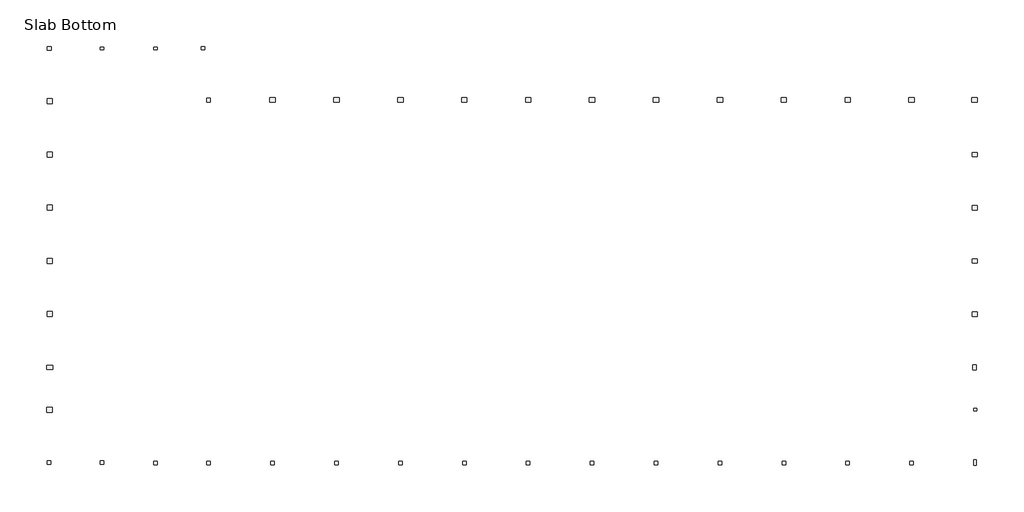
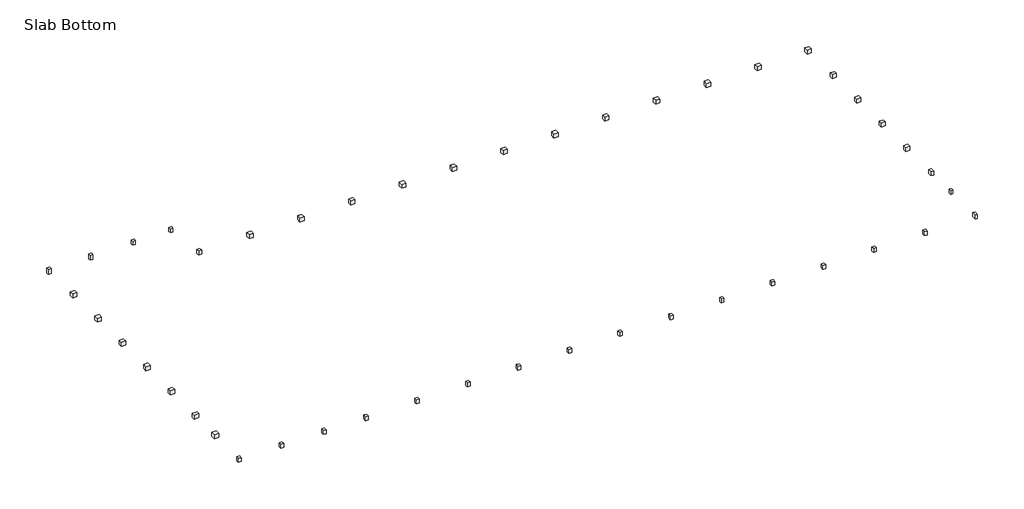
# One storey: 46 slabs.
"""IFC4 building model written with IfcOpenShell, lengths in millimetres."""

from ifc_helpers import new_model, si_unit, frame, origin, place, context, project, spatial, polyline, outline, extrude, faceted_brep, element, save

model = new_model("IFC4")

# Units and contexts
model_context = context("Model", 3, world=origin())
ifc_project = project(units=[si_unit("LENGTHUNIT", "METRE", prefix="MILLI")], contexts=[model_context])

# Site, building, storey
site = spatial("IfcSite", under=ifc_project)
building = spatial("IfcBuilding", under=site)
storey = spatial("IfcBuildingStorey", under=building, Name="Slab Bottom", Elevation=-152.4)

# Slabs
placement = place(None, origin())
element("IfcSlab", 1, ObjectType="Footing-Rectangular : P1", at=placement, inside=storey, context=model_context, shape_type="SweptSolid", body=[
    extrude(outline(polyline([(411310.2398264, -572441.1413841), (411615.0398264, -572441.1413841), (411615.0398264, -572745.9413841), (411310.2398264, -572745.9413841), (411310.2398264, -572441.1413841)])), frame((0.0, 0.0, -914.4), z_axis=(0.0, 0.0, 1.0), x_axis=(1.0, 0.0, 0.0)), (0.0, 0.0, 1.0), 609.6),
])
element("IfcSlab", 2, ObjectType="Footing-Rectangular : P10", at=placement, inside=storey, context=model_context, shape_type="SweptSolid", body=[
    extrude(outline(polyline([(304585.7898264, -567919.9413841), (304585.7898264, -567462.7413841), (305271.5898264, -567462.7413841), (305271.5898264, -567919.9413841), (304585.7898264, -567919.9413841)])), frame((0.0, 0.0, -914.4), z_axis=(0.0, 0.0, 1.0), x_axis=(1.0, 0.0, 0.0)), (0.0, 0.0, 1.0), 609.6),
])
element("IfcSlab", 3, ObjectType="Footing-Rectangular : P11", at=placement, inside=storey, context=model_context, shape_type="SweptSolid", body=[
    extrude(outline(polyline([(411138.7898264, -549562.0913841), (411138.7898264, -549054.0913841), (411697.5898264, -549054.0913841), (411697.5898264, -549562.0913841), (411138.7898264, -549562.0913841)])), frame((0.0, 0.0, -914.4), z_axis=(0.0, 0.0, 1.0), x_axis=(1.0, 0.0, 0.0)), (0.0, 0.0, 1.0), 609.6),
])
element("IfcSlab", 4, ObjectType="Footing-Rectangular : P11A", at=placement, inside=storey, context=model_context, shape_type="SweptSolid", body=[
    extrude(outline(polyline([(411138.7898264, -561817.5913841), (411138.7898264, -561309.5913841), (411697.5898264, -561309.5913841), (411697.5898264, -561817.5913841), (411138.7898264, -561817.5913841)])), frame((0.0, 0.0, -914.4), z_axis=(0.0, 0.0, 1.0), x_axis=(1.0, 0.0, 0.0)), (0.0, 0.0, 1.0), 609.6),
])
element("IfcSlab", 5, ObjectType="Footing-Rectangular : P12", at=placement, inside=storey, context=model_context, shape_type="SweptSolid", body=[
    extrude(outline(polyline([(304649.2898264, -537331.9913841), (304649.2898264, -536773.1913841), (305258.8898264, -536773.1913841), (305258.8898264, -537331.9913841), (304649.2898264, -537331.9913841)])), frame((0.0, 0.0, -914.4), z_axis=(0.0, 0.0, 1.0), x_axis=(1.0, 0.0, 0.0)), (0.0, 0.0, 1.0), 609.6),
])
element("IfcSlab", 6, ObjectType="Footing-Rectangular : P12", at=placement, inside=storey, context=model_context, shape_type="SweptSolid", body=[
    extrude(outline(polyline([(304649.2898264, -543459.7413841), (304649.2898264, -542900.9413841), (305258.8898264, -542900.9413841), (305258.8898264, -543459.7413841), (304649.2898264, -543459.7413841)])), frame((0.0, 0.0, -914.4), z_axis=(0.0, 0.0, 1.0), x_axis=(1.0, 0.0, 0.0)), (0.0, 0.0, 1.0), 609.6),
])
element("IfcSlab", 7, ObjectType="Footing-Rectangular : P12", at=placement, inside=storey, context=model_context, shape_type="SweptSolid", body=[
    extrude(outline(polyline([(304649.2898264, -549587.4913841), (304649.2898264, -549028.6913841), (305258.8898264, -549028.6913841), (305258.8898264, -549587.4913841), (304649.2898264, -549587.4913841)])), frame((0.0, 0.0, -914.4), z_axis=(0.0, 0.0, 1.0), x_axis=(1.0, 0.0, 0.0)), (0.0, 0.0, 1.0), 609.6),
])
element("IfcSlab", 8, ObjectType="Footing-Rectangular : P12", at=placement, inside=storey, context=model_context, shape_type="SweptSolid", body=[
    extrude(outline(polyline([(304649.2898264, -555715.2413841), (304649.2898264, -555156.4413841), (305258.8898264, -555156.4413841), (305258.8898264, -555715.2413841), (304649.2898264, -555715.2413841)])), frame((0.0, 0.0, -914.4), z_axis=(0.0, 0.0, 1.0), x_axis=(1.0, 0.0, 0.0)), (0.0, 0.0, 1.0), 609.6),
])
element("IfcSlab", 9, ObjectType="Footing-Rectangular : P12", at=placement, inside=storey, context=model_context, shape_type="SweptSolid", body=[
    extrude(outline(polyline([(304649.2898264, -561842.9913841), (304649.2898264, -561284.1913841), (305258.8898264, -561284.1913841), (305258.8898264, -561842.9913841), (304649.2898264, -561842.9913841)])), frame((0.0, 0.0, -914.4), z_axis=(0.0, 0.0, 1.0), x_axis=(1.0, 0.0, 0.0)), (0.0, 0.0, 1.0), 609.6),
])
element("IfcSlab", 10, ObjectType="Footing-Rectangular : P13", at=placement, inside=storey, context=model_context, shape_type="SweptSolid", body=[
    extrude(outline(polyline([(396476.6398264, -536627.1413358), (397086.2398264, -536627.1413358), (397086.2398264, -537185.9413358), (396476.6398264, -537185.9413358), (396476.6398264, -536627.1413358)])), frame((0.0, 0.0, -914.4), z_axis=(0.0, 0.0, 1.0), x_axis=(1.0, 0.0, 0.0)), (0.0, 0.0, 1.0), 609.6),
])
element("IfcSlab", 11, ObjectType="Footing-Rectangular : P13", at=placement, inside=storey, context=model_context, shape_type="SweptSolid", body=[
    extrude(outline(polyline([(389123.3398264, -536627.1413358), (389732.9398264, -536627.1413358), (389732.9398264, -537185.9413358), (389123.3398264, -537185.9413358), (389123.3398264, -536627.1413358)])), frame((0.0, 0.0, -914.4), z_axis=(0.0, 0.0, 1.0), x_axis=(1.0, 0.0, 0.0)), (0.0, 0.0, 1.0), 609.6),
])
element("IfcSlab", 12, ObjectType="Footing-Rectangular : P13", at=placement, inside=storey, context=model_context, shape_type="SweptSolid", body=[
    extrude(outline(polyline([(381770.0398264, -536627.1413358), (382379.6398264, -536627.1413358), (382379.6398264, -537185.9413358), (381770.0398264, -537185.9413358), (381770.0398264, -536627.1413358)])), frame((0.0, 0.0, -914.4), z_axis=(0.0, 0.0, 1.0), x_axis=(1.0, 0.0, 0.0)), (0.0, 0.0, 1.0), 609.6),
])
element("IfcSlab", 13, ObjectType="Footing-Rectangular : P13", at=placement, inside=storey, context=model_context, shape_type="SweptSolid", body=[
    extrude(outline(polyline([(374416.7398264, -536627.1413358), (375026.3398264, -536627.1413358), (375026.3398264, -537185.9413358), (374416.7398264, -537185.9413358), (374416.7398264, -536627.1413358)])), frame((0.0, 0.0, -914.4), z_axis=(0.0, 0.0, 1.0), x_axis=(1.0, 0.0, 0.0)), (0.0, 0.0, 1.0), 609.6),
])
element("IfcSlab", 14, ObjectType="Footing-Rectangular : P13", at=placement, inside=storey, context=model_context, shape_type="SweptSolid", body=[
    extrude(outline(polyline([(367063.4398264, -536627.1413358), (367673.0398264, -536627.1413358), (367673.0398264, -537185.9413358), (367063.4398264, -537185.9413358), (367063.4398264, -536627.1413358)])), frame((0.0, 0.0, -914.4), z_axis=(0.0, 0.0, 1.0), x_axis=(1.0, 0.0, 0.0)), (0.0, 0.0, 1.0), 609.6),
])
element("IfcSlab", 15, ObjectType="Footing-Rectangular : P13", at=placement, inside=storey, context=model_context, shape_type="SweptSolid", body=[
    extrude(outline(polyline([(359710.1398264, -536627.1413358), (360319.7398264, -536627.1413358), (360319.7398264, -537185.9413358), (359710.1398264, -537185.9413358), (359710.1398264, -536627.1413358)])), frame((0.0, 0.0, -914.4), z_axis=(0.0, 0.0, 1.0), x_axis=(1.0, 0.0, 0.0)), (0.0, 0.0, 1.0), 609.6),
])
element("IfcSlab", 16, ObjectType="Footing-Rectangular : P13", at=placement, inside=storey, context=model_context, shape_type="SweptSolid", body=[
    extrude(outline(polyline([(352356.8398264, -536627.1413358), (352966.4398264, -536627.1413358), (352966.4398264, -537185.9413358), (352356.8398264, -537185.9413358), (352356.8398264, -536627.1413358)])), frame((0.0, 0.0, -914.4), z_axis=(0.0, 0.0, 1.0), x_axis=(1.0, 0.0, 0.0)), (0.0, 0.0, 1.0), 609.6),
])
element("IfcSlab", 17, ObjectType="Footing-Rectangular : P13", at=placement, inside=storey, context=model_context, shape_type="SweptSolid", body=[
    extrude(outline(polyline([(345003.5398264, -536627.1413358), (345613.1398264, -536627.1413358), (345613.1398264, -537185.9413358), (345003.5398264, -537185.9413358), (345003.5398264, -536627.1413358)])), frame((0.0, 0.0, -914.4), z_axis=(0.0, 0.0, 1.0), x_axis=(1.0, 0.0, 0.0)), (0.0, 0.0, 1.0), 609.6),
])
element("IfcSlab", 18, ObjectType="Footing-Rectangular : P13", at=placement, inside=storey, context=model_context, shape_type="SweptSolid", body=[
    extrude(outline(polyline([(337650.2398264, -536627.1413358), (338259.8398264, -536627.1413358), (338259.8398264, -537185.9413358), (337650.2398264, -537185.9413358), (337650.2398264, -536627.1413358)])), frame((0.0, 0.0, -914.4), z_axis=(0.0, 0.0, 1.0), x_axis=(1.0, 0.0, 0.0)), (0.0, 0.0, 1.0), 609.6),
])
element("IfcSlab", 19, ObjectType="Footing-Rectangular : P13", at=placement, inside=storey, context=model_context, shape_type="SweptSolid", body=[
    extrude(outline(polyline([(330296.9398264, -536627.1413358), (330906.5398264, -536627.1413358), (330906.5398264, -537185.9413358), (330296.9398264, -537185.9413358), (330296.9398264, -536627.1413358)])), frame((0.0, 0.0, -914.4), z_axis=(0.0, 0.0, 1.0), x_axis=(1.0, 0.0, 0.0)), (0.0, 0.0, 1.0), 609.6),
])
element("IfcSlab", 20, ObjectType="Footing-Rectangular : P13A", at=placement, inside=storey, context=model_context, shape_type="SweptSolid", body=[
    extrude(outline(polyline([(411081.6397781, -536620.7913358), (411691.2397781, -536620.7913358), (411691.2397781, -537179.5913358), (411081.6397781, -537179.5913358), (411081.6397781, -536620.7913358)])), frame((0.0, 0.0, -914.4), z_axis=(0.0, 0.0, 1.0), x_axis=(1.0, 0.0, 0.0)), (0.0, 0.0, 1.0), 609.6),
])
element("IfcSlab", 21, ObjectType="Footing-Rectangular : P13B", at=placement, inside=storey, context=model_context, shape_type="SweptSolid", body=[
    extrude(outline(polyline([(403829.9398264, -536627.1413358), (404439.5398264, -536627.1413358), (404439.5398264, -537185.9413358), (403829.9398264, -537185.9413358), (403829.9398264, -536627.1413358)])), frame((0.0, 0.0, -914.4), z_axis=(0.0, 0.0, 1.0), x_axis=(1.0, 0.0, 0.0)), (0.0, 0.0, 1.0), 609.6),
])
element("IfcSlab", 22, ObjectType="Footing-Rectangular : P14", at=placement, inside=storey, context=model_context, shape_type="Brep", body=[
    faceted_brep([(304598.4898264, -572288.7413841, -304.8), (304598.4898264, -572898.3413841, -304.8), (305258.8898264, -572898.3413841, -304.8), (305258.8898264, -572810.8391729, -304.8), (305258.8898264, -572404.4391729, -304.8), (305258.8898264, -572288.7413841, -304.8), (304598.4898264, -572288.7413841, -914.4), (304598.4898264, -572898.3413841, -914.4), (305258.8898264, -572898.3413841, -914.4), (305258.8898264, -572288.7413841, -914.4)], [[[0, 1, 2, 3, 4, 5]], [[1, 0, 6, 7]], [[2, 1, 7, 8]], [[5, 4, 3, 2, 8, 9]], [[0, 5, 9, 6]], [[7, 6, 9, 8]]]),
])
element("IfcSlab", 23, ObjectType="Footing-Rectangular : P2", at=placement, inside=storey, context=model_context, shape_type="SweptSolid", body=[
    extrude(outline(polyline([(322772.1898264, -530797.8413841), (322772.1898264, -531102.6413841), (322365.7898264, -531102.6413841), (322365.7898264, -530797.8413841), (322772.1898264, -530797.8413841)])), frame((0.0, 0.0, -914.4), z_axis=(0.0, 0.0, 1.0), x_axis=(1.0, 0.0, 0.0)), (0.0, 0.0, 1.0), 609.6),
])
element("IfcSlab", 24, ObjectType="Footing-Rectangular : P3", at=placement, inside=storey, context=model_context, shape_type="SweptSolid", body=[
    extrude(outline(polyline([(411284.8398264, -578384.7413841), (411589.6398264, -578384.7413841), (411589.6398264, -578994.3413841), (411284.8398264, -578994.3413841), (411284.8398264, -578384.7413841)])), frame((0.0, 0.0, -914.4), z_axis=(0.0, 0.0, 1.0), x_axis=(1.0, 0.0, 0.0)), (0.0, 0.0, 1.0), 609.6),
])
element("IfcSlab", 25, ObjectType="Footing-Rectangular : P4", at=placement, inside=storey, context=model_context, shape_type="SweptSolid", body=[
    extrude(outline(polyline([(310789.7398264, -531108.9913841), (310789.7398264, -530804.1913841), (311196.1398264, -530804.1913841), (311196.1398264, -531108.9913841), (310789.7398264, -531108.9913841)])), frame((0.0, 0.0, -1066.8), z_axis=(0.0, 0.0, 1.0), x_axis=(1.0, 0.0, 0.0)), (0.0, 0.0, 1.0), 762.0),
])
element("IfcSlab", 26, ObjectType="Footing-Rectangular : P4", at=placement, inside=storey, context=model_context, shape_type="SweptSolid", body=[
    extrude(outline(polyline([(317323.8898264, -531108.9913841), (316917.4898264, -531108.9913841), (316917.4898264, -530804.1913841), (317323.8898264, -530804.1913841), (317323.8898264, -531108.9913841)])), frame((0.0, 0.0, -914.4), z_axis=(0.0, 0.0, 1.0), x_axis=(1.0, 0.0, 0.0)), (0.0, 0.0, 1.0), 609.6),
])
element("IfcSlab", 27, ObjectType="Footing-Rectangular : P5", at=placement, inside=storey, context=model_context, shape_type="SweptSolid", body=[
    extrude(outline(polyline([(330398.5398264, -578537.1413841), (330804.9398264, -578537.1413841), (330804.9398264, -578943.5413841), (330398.5398264, -578943.5413841), (330398.5398264, -578537.1413841)])), frame((0.0, 0.0, -914.4), z_axis=(0.0, 0.0, 1.0), x_axis=(1.0, 0.0, 0.0)), (0.0, 0.0, 1.0), 609.6),
])
element("IfcSlab", 28, ObjectType="Footing-Rectangular : P5", at=placement, inside=storey, context=model_context, shape_type="SweptSolid", body=[
    extrude(outline(polyline([(337751.8398264, -578537.1413841), (338158.2398264, -578537.1413841), (338158.2398264, -578943.5413841), (337751.8398264, -578943.5413841), (337751.8398264, -578537.1413841)])), frame((0.0, 0.0, -914.4), z_axis=(0.0, 0.0, 1.0), x_axis=(1.0, 0.0, 0.0)), (0.0, 0.0, 1.0), 609.6),
])
element("IfcSlab", 29, ObjectType="Footing-Rectangular : P5", at=placement, inside=storey, context=model_context, shape_type="SweptSolid", body=[
    extrude(outline(polyline([(345105.1398264, -578537.1413841), (345511.5398264, -578537.1413841), (345511.5398264, -578943.5413841), (345105.1398264, -578943.5413841), (345105.1398264, -578537.1413841)])), frame((0.0, 0.0, -914.4), z_axis=(0.0, 0.0, 1.0), x_axis=(1.0, 0.0, 0.0)), (0.0, 0.0, 1.0), 609.6),
])
element("IfcSlab", 30, ObjectType="Footing-Rectangular : P5", at=placement, inside=storey, context=model_context, shape_type="SweptSolid", body=[
    extrude(outline(polyline([(352458.4398264, -578537.1413841), (352864.8398264, -578537.1413841), (352864.8398264, -578943.5413841), (352458.4398264, -578943.5413841), (352458.4398264, -578537.1413841)])), frame((0.0, 0.0, -914.4), z_axis=(0.0, 0.0, 1.0), x_axis=(1.0, 0.0, 0.0)), (0.0, 0.0, 1.0), 609.6),
])
element("IfcSlab", 31, ObjectType="Footing-Rectangular : P5", at=placement, inside=storey, context=model_context, shape_type="SweptSolid", body=[
    extrude(outline(polyline([(359811.7398264, -578537.1413841), (360218.1398264, -578537.1413841), (360218.1398264, -578943.5413841), (359811.7398264, -578943.5413841), (359811.7398264, -578537.1413841)])), frame((0.0, 0.0, -914.4), z_axis=(0.0, 0.0, 1.0), x_axis=(1.0, 0.0, 0.0)), (0.0, 0.0, 1.0), 609.6),
])
element("IfcSlab", 32, ObjectType="Footing-Rectangular : P5", at=placement, inside=storey, context=model_context, shape_type="SweptSolid", body=[
    extrude(outline(polyline([(367165.0398264, -578537.1413841), (367571.4398264, -578537.1413841), (367571.4398264, -578943.5413841), (367165.0398264, -578943.5413841), (367165.0398264, -578537.1413841)])), frame((0.0, 0.0, -914.4), z_axis=(0.0, 0.0, 1.0), x_axis=(1.0, 0.0, 0.0)), (0.0, 0.0, 1.0), 609.6),
])
element("IfcSlab", 33, ObjectType="Footing-Rectangular : P5", at=placement, inside=storey, context=model_context, shape_type="SweptSolid", body=[
    extrude(outline(polyline([(374518.3398264, -578537.1413841), (374924.7398264, -578537.1413841), (374924.7398264, -578943.5413841), (374518.3398264, -578943.5413841), (374518.3398264, -578537.1413841)])), frame((0.0, 0.0, -914.4), z_axis=(0.0, 0.0, 1.0), x_axis=(1.0, 0.0, 0.0)), (0.0, 0.0, 1.0), 609.6),
])
element("IfcSlab", 34, ObjectType="Footing-Rectangular : P5", at=placement, inside=storey, context=model_context, shape_type="SweptSolid", body=[
    extrude(outline(polyline([(381871.6398264, -578537.1413841), (382278.0398264, -578537.1413841), (382278.0398264, -578943.5413841), (381871.6398264, -578943.5413841), (381871.6398264, -578537.1413841)])), frame((0.0, 0.0, -914.4), z_axis=(0.0, 0.0, 1.0), x_axis=(1.0, 0.0, 0.0)), (0.0, 0.0, 1.0), 609.6),
])
element("IfcSlab", 35, ObjectType="Footing-Rectangular : P5", at=placement, inside=storey, context=model_context, shape_type="SweptSolid", body=[
    extrude(outline(polyline([(389224.9398264, -578537.1413841), (389631.3398264, -578537.1413841), (389631.3398264, -578943.5413841), (389224.9398264, -578943.5413841), (389224.9398264, -578537.1413841)])), frame((0.0, 0.0, -914.4), z_axis=(0.0, 0.0, 1.0), x_axis=(1.0, 0.0, 0.0)), (0.0, 0.0, 1.0), 609.6),
])
element("IfcSlab", 36, ObjectType="Footing-Rectangular : P5A", at=placement, inside=storey, context=model_context, shape_type="SweptSolid", body=[
    extrude(outline(polyline([(317327.0648264, -578937.1913841), (316920.6648264, -578937.1913841), (316920.6648264, -578530.7913841), (317327.0648264, -578530.7913841), (317327.0648264, -578937.1913841)])), frame((0.0, 0.0, -914.4), z_axis=(0.0, 0.0, 1.0), x_axis=(1.0, 0.0, 0.0)), (0.0, 0.0, 1.0), 609.6),
])
element("IfcSlab", 37, ObjectType="Footing-Rectangular : P5A", at=placement, inside=storey, context=model_context, shape_type="SweptSolid", body=[
    extrude(outline(polyline([(323016.6648264, -578937.1913841), (323016.6648264, -578530.7913841), (323423.0648264, -578530.7913841), (323423.0648264, -578937.1913841), (323016.6648264, -578937.1913841)])), frame((0.0, 0.0, -914.4), z_axis=(0.0, 0.0, 1.0), x_axis=(1.0, 0.0, 0.0)), (0.0, 0.0, 1.0), 609.6),
])
element("IfcSlab", 38, ObjectType="Footing-Rectangular : P5A", at=placement, inside=storey, context=model_context, shape_type="SweptSolid", body=[
    extrude(outline(polyline([(396578.2398264, -578530.7913841), (396984.6398264, -578530.7913841), (396984.6398264, -578937.1913841), (396578.2398264, -578937.1913841), (396578.2398264, -578530.7913841)])), frame((0.0, 0.0, -914.4), z_axis=(0.0, 0.0, 1.0), x_axis=(1.0, 0.0, 0.0)), (0.0, 0.0, 1.0), 609.6),
])
element("IfcSlab", 39, ObjectType="Footing-Rectangular : P5A", at=placement, inside=storey, context=model_context, shape_type="SweptSolid", body=[
    extrude(outline(polyline([(403931.5398264, -578530.7913841), (404337.9398264, -578530.7913841), (404337.9398264, -578937.1913841), (403931.5398264, -578937.1913841), (403931.5398264, -578530.7913841)])), frame((0.0, 0.0, -914.4), z_axis=(0.0, 0.0, 1.0), x_axis=(1.0, 0.0, 0.0)), (0.0, 0.0, 1.0), 609.6),
])
element("IfcSlab", 40, ObjectType="Footing-Rectangular : P5B", at=placement, inside=storey, context=model_context, shape_type="SweptSolid", body=[
    extrude(outline(polyline([(311196.1398264, -578892.7413841), (310789.7398264, -578892.7413841), (310789.7398264, -578486.3413841), (311196.1398264, -578486.3413841), (311196.1398264, -578892.7413841)])), frame((0.0, 0.0, -914.4), z_axis=(0.0, 0.0, 1.0), x_axis=(1.0, 0.0, 0.0)), (0.0, 0.0, 1.0), 609.6),
])
element("IfcSlab", 41, ObjectType="Footing-Rectangular : P5C", at=placement, inside=storey, context=model_context, shape_type="SweptSolid", body=[
    extrude(outline(polyline([(304642.9398264, -578899.0913841), (304642.9398264, -578492.6913841), (305049.3398264, -578492.6913841), (305049.3398264, -578899.0913841), (304642.9398264, -578899.0913841)])), frame((0.0, 0.0, -914.4), z_axis=(0.0, 0.0, 1.0), x_axis=(1.0, 0.0, 0.0)), (0.0, 0.0, 1.0), 609.6),
])
element("IfcSlab", 42, ObjectType="Footing-Rectangular : P6", at=placement, inside=storey, context=model_context, shape_type="SweptSolid", body=[
    extrude(outline(polyline([(323019.8398264, -536677.9413841), (323426.2398264, -536677.9413841), (323426.2398264, -537135.1413841), (323019.8398264, -537135.1413841), (323019.8398264, -536677.9413841)])), frame((0.0, 0.0, -914.4), z_axis=(0.0, 0.0, 1.0), x_axis=(1.0, 0.0, 0.0)), (0.0, 0.0, 1.0), 609.6),
])
element("IfcSlab", 43, ObjectType="Footing-Rectangular : P6A", at=placement, inside=storey, context=model_context, shape_type="SweptSolid", body=[
    extrude(outline(polyline([(304681.0398264, -530747.0413841), (305138.2398264, -530747.0413841), (305138.2398264, -531153.4413841), (304681.0398264, -531153.4413841), (304681.0398264, -530747.0413841)])), frame((0.0, 0.0, -1066.8), z_axis=(0.0, 0.0, 1.0), x_axis=(1.0, 0.0, 0.0)), (0.0, 0.0, 1.0), 762.0),
])
element("IfcSlab", 44, ObjectType="Footing-Rectangular : P7", at=placement, inside=storey, context=model_context, shape_type="SweptSolid", body=[
    extrude(outline(polyline([(411183.2398264, -567424.6413841), (411589.6398264, -567424.6413841), (411589.6398264, -567983.4413841), (411183.2398264, -567983.4413841), (411183.2398264, -567424.6413841)])), frame((0.0, 0.0, -914.4), z_axis=(0.0, 0.0, 1.0), x_axis=(1.0, 0.0, 0.0)), (0.0, 0.0, 1.0), 609.6),
])
element("IfcSlab", 45, ObjectType="Footing-Rectangular : P8", at=placement, inside=storey, context=model_context, shape_type="SweptSolid", body=[
    extrude(outline(polyline([(411138.7898264, -555664.4413841), (411138.7898264, -555207.2413841), (411697.5898264, -555207.2413841), (411697.5898264, -555664.4413841), (411138.7898264, -555664.4413841)])), frame((0.0, 0.0, -914.4), z_axis=(0.0, 0.0, 1.0), x_axis=(1.0, 0.0, 0.0)), (0.0, 0.0, 1.0), 609.6),
])
element("IfcSlab", 46, ObjectType="Footing-Rectangular : P9", at=placement, inside=storey, context=model_context, shape_type="SweptSolid", body=[
    extrude(outline(polyline([(411107.0398264, -543408.9413841), (411107.0398264, -542951.7413841), (411716.6398264, -542951.7413841), (411716.6398264, -543408.9413841), (411107.0398264, -543408.9413841)])), frame((0.0, 0.0, -914.4), z_axis=(0.0, 0.0, 1.0), x_axis=(1.0, 0.0, 0.0)), (0.0, 0.0, 1.0), 609.6),
])

save(model, "model.ifc")

# Revit data of these elements
# Type "Footing-Rectangular : P1"
#   Type Mark = ""
#   Assembly Code = "A1010100"
#   Width = 1' - 0"
#   Length = 1' - 0"
#   Thickness = 2' - 6"
#   Structural Material [instance default] = Concrete, Cast-in-Place gray
# Type "Footing-Rectangular : P10"
#   Assembly Code = "A1010100"
#   Width = 1' - 6"
#   Length = 2' - 3"
#   Thickness = 2' - 6"
#   Structural Material [instance default] = Concrete, Cast-in-Place gray
# Type "Footing-Rectangular : P11"
#   Assembly Code = "A1010100"
#   Width = 1' - 8"
#   Length = 1' - 10"
#   Thickness = 2' - 6"
#   Structural Material [instance default] = Concrete, Cast-in-Place gray
# Type "Footing-Rectangular : P11A"
#   Assembly Code = "A1010100"
#   Width = 1' - 8"
#   Length = 1' - 10"
#   Thickness = 2' - 6"
#   Structural Material [instance default] = Concrete, Cast-in-Place gray
# Type "Footing-Rectangular : P12"
#   Assembly Code = "A1010100"
#   Width = 1' - 10"
#   Length = 2' - 0"
#   Thickness = 2' - 6"
#   Structural Material [instance default] = Concrete, Cast-in-Place gray
# Type "Footing-Rectangular : P13"
#   Assembly Code = "A1010100"
#   Width = 2' - 0"
#   Length = 1' - 10"
#   Thickness = 2' - 6"
#   Structural Material [instance default] = Concrete, Cast-in-Place gray
# Type "Footing-Rectangular : P13A"
#   Assembly Code = "A1010100"
#   Width = 2' - 0"
#   Length = 1' - 10"
#   Thickness = 2' - 6"
#   Structural Material [instance default] = Concrete, Cast-in-Place gray
# Type "Footing-Rectangular : P13B"
#   Assembly Code = "A1010100"
#   Width = 2' - 0"
#   Length = 1' - 10"
#   Thickness = 2' - 6"
#   Structural Material [instance default] = Concrete, Cast-in-Place gray
# Type "Footing-Rectangular : P14"
#   Assembly Code = "A1010100"
#   Width = 2' - 0"
#   Length = 2' - 2"
#   Thickness = 2' - 6"
#   Structural Material [instance default] = Concrete, Cast-in-Place gray
# Type "Footing-Rectangular : P2"
#   Assembly Code = "A1010100"
#   Width = 1' - 0"
#   Length = 1' - 4"
#   Thickness = 2' - 6"
#   Structural Material [instance default] = Concrete, Cast-in-Place gray
# Type "Footing-Rectangular : P3"
#   Assembly Code = "A1010100"
#   Width = 1' - 0"
#   Length = 2' - 0"
#   Thickness = 2' - 6"
#   Structural Material [instance default] = Concrete, Cast-in-Place gray
# Type "Footing-Rectangular : P4"
#   Assembly Code = "A1010100"
#   Width = 1' - 4"
#   Length = 1' - 0"
#   Thickness = 2' - 6"
#   Structural Material [instance default] = Concrete, Cast-in-Place gray
# Type "Footing-Rectangular : P5"
#   Assembly Code = "A1010100"
#   Width = 1' - 4"
#   Length = 1' - 4"
#   Thickness = 2' - 6"
#   Structural Material [instance default] = Concrete, Cast-in-Place gray
# Type "Footing-Rectangular : P5A"
#   Assembly Code = "A1010100"
#   Width = 1' - 4"
#   Length = 1' - 4"
#   Thickness = 2' - 6"
#   Structural Material [instance default] = Concrete, Cast-in-Place gray
# Type "Footing-Rectangular : P5B"
#   Assembly Code = "A1010100"
#   Width = 1' - 4"
#   Length = 1' - 4"
#   Thickness = 2' - 6"
#   Structural Material [instance default] = Concrete, Cast-in-Place gray
# Type "Footing-Rectangular : P5C"
#   Assembly Code = "A1010100"
#   Width = 1' - 4"
#   Length = 1' - 4"
#   Thickness = 2' - 6"
#   Structural Material [instance default] = Concrete, Cast-in-Place gray
# Type "Footing-Rectangular : P6"
#   Assembly Code = "A1010100"
#   Width = 1' - 4"
#   Length = 1' - 6"
#   Thickness = 2' - 6"
#   Structural Material [instance default] = Concrete, Cast-in-Place gray
# Type "Footing-Rectangular : P6A"
#   Assembly Code = "A1010100"
#   Width = 1' - 4"
#   Length = 1' - 6"
#   Thickness = 2' - 6"
#   Structural Material [instance default] = Concrete, Cast-in-Place gray
# Type "Footing-Rectangular : P7"
#   Assembly Code = "A1010100"
#   Width = 1' - 4"
#   Length = 1' - 10"
#   Thickness = 2' - 6"
#   Structural Material [instance default] = Concrete, Cast-in-Place gray
# Type "Footing-Rectangular : P8"
#   Assembly Code = "A1010100"
#   Width = 1' - 6"
#   Length = 1' - 10"
#   Thickness = 2' - 6"
#   Structural Material [instance default] = Concrete, Cast-in-Place gray
# Type "Footing-Rectangular : P9"
#   Assembly Code = "A1010100"
#   Width = 1' - 6"
#   Length = 2' - 0"
#   Thickness = 2' - 6"
#   Structural Material [instance default] = Concrete, Cast-in-Place gray
# Element 1 (IfcSlab, "Footing-Rectangular : P1")
#   Comments = ""
#   Structural Material = Concrete, Cast-in-Place gray
#   Phase Created = New Construction
#   Materials on its faces: "Concrete, Cast-in-Place gray"
# Element 2 (IfcSlab, "Footing-Rectangular : P10")
#   Comments = ""
#   Structural Material = Concrete, Cast-in-Place gray
#   Phase Created = New Construction
#   Materials on its faces: "Concrete, Cast-in-Place gray"
# Element 3 (IfcSlab, "Footing-Rectangular : P11")
#   Comments = ""
#   Structural Material = Concrete, Cast-in-Place gray
#   Phase Created = New Construction
#   Materials on its faces: "Concrete, Cast-in-Place gray"
# Element 4 (IfcSlab, "Footing-Rectangular : P11A")
#   Comments = ""
#   Structural Material = Concrete, Cast-in-Place gray
#   Phase Created = New Construction
#   Materials on its faces: "Concrete, Cast-in-Place gray"
# Elements 5, 6, 7, 8, 9 (IfcSlab, "Footing-Rectangular : P12")
#   Comments = ""
#   Structural Material = Concrete, Cast-in-Place gray
#   Phase Created = New Construction
#   Materials on its faces: "Concrete, Cast-in-Place gray"
# Elements 10, 11, 12, 13, 14, 15, 16, 17, 18, 19 (IfcSlab, "Footing-Rectangular : P13")
#   Comments = ""
#   Structural Material = Concrete, Cast-in-Place gray
#   Phase Created = New Construction
#   Materials on its faces: "Concrete, Cast-in-Place gray"
# Element 20 (IfcSlab, "Footing-Rectangular : P13A")
#   Comments = ""
#   Structural Material = Concrete, Cast-in-Place gray
#   Phase Created = New Construction
#   Materials on its faces: "Concrete, Cast-in-Place gray"
# Element 21 (IfcSlab, "Footing-Rectangular : P13B")
#   Comments = ""
#   Structural Material = Concrete, Cast-in-Place gray
#   Phase Created = New Construction
#   Materials on its faces: "Concrete, Cast-in-Place gray"
# Element 22 (IfcSlab, "Footing-Rectangular : P14")
#   Comments = ""
#   Structural Material = Concrete, Cast-in-Place gray
#   Phase Created = New Construction
#   Materials on its faces: "Concrete, Cast-in-Place gray"
# Element 23 (IfcSlab, "Footing-Rectangular : P2")
#   Comments = ""
#   Structural Material = Concrete, Cast-in-Place gray
#   Phase Created = New Construction
#   Materials on its faces: "Concrete, Cast-in-Place gray"
# Element 24 (IfcSlab, "Footing-Rectangular : P3")
#   Comments = ""
#   Structural Material = Concrete, Cast-in-Place gray
#   Phase Created = New Construction
#   Materials on its faces: "Concrete, Cast-in-Place gray"
# Elements 25, 26 (IfcSlab, "Footing-Rectangular : P4")
#   Comments = ""
#   Structural Material = Concrete, Cast-in-Place gray
#   Phase Created = New Construction
#   Materials on its faces: "Concrete, Cast-in-Place gray"
# Elements 27, 28, 29, 30, 31, 32, 33, 34, 35 (IfcSlab, "Footing-Rectangular : P5")
#   Comments = ""
#   Structural Material = Concrete, Cast-in-Place gray
#   Phase Created = New Construction
#   Materials on its faces: "Concrete, Cast-in-Place gray"
# Elements 36, 37, 38, 39 (IfcSlab, "Footing-Rectangular : P5A")
#   Comments = ""
#   Structural Material = Concrete, Cast-in-Place gray
#   Phase Created = New Construction
#   Materials on its faces: "Concrete, Cast-in-Place gray"
# Element 40 (IfcSlab, "Footing-Rectangular : P5B")
#   Comments = ""
#   Structural Material = Concrete, Cast-in-Place gray
#   Phase Created = New Construction
#   Materials on its faces: "Concrete, Cast-in-Place gray"
# Element 41 (IfcSlab, "Footing-Rectangular : P5C")
#   Comments = ""
#   Structural Material = Concrete, Cast-in-Place gray
#   Phase Created = New Construction
#   Materials on its faces: "Concrete, Cast-in-Place gray"
# Element 42 (IfcSlab, "Footing-Rectangular : P6")
#   Comments = ""
#   Structural Material = Concrete, Cast-in-Place gray
#   Phase Created = New Construction
#   Materials on its faces: "Concrete, Cast-in-Place gray"
# Element 43 (IfcSlab, "Footing-Rectangular : P6A")
#   Comments = ""
#   Structural Material = Concrete, Cast-in-Place gray
#   Phase Created = New Construction
#   Materials on its faces: "Concrete, Cast-in-Place gray"
# Element 44 (IfcSlab, "Footing-Rectangular : P7")
#   Comments = ""
#   Structural Material = Concrete, Cast-in-Place gray
#   Phase Created = New Construction
#   Materials on its faces: "Concrete, Cast-in-Place gray"
# Element 45 (IfcSlab, "Footing-Rectangular : P8")
#   Comments = ""
#   Structural Material = Concrete, Cast-in-Place gray
#   Phase Created = New Construction
#   Materials on its faces: "Concrete, Cast-in-Place gray"
# Element 46 (IfcSlab, "Footing-Rectangular : P9")
#   Comments = ""
#   Structural Material = Concrete, Cast-in-Place gray
#   Phase Created = New Construction
#   Materials on its faces: "Concrete, Cast-in-Place gray"
# Materials
#   "Concrete, Cast-in-Place gray": class "Concrete", colour RGB 192 192 192, transparency 0, Description = "Cast-in-place concrete", Cost = 0
